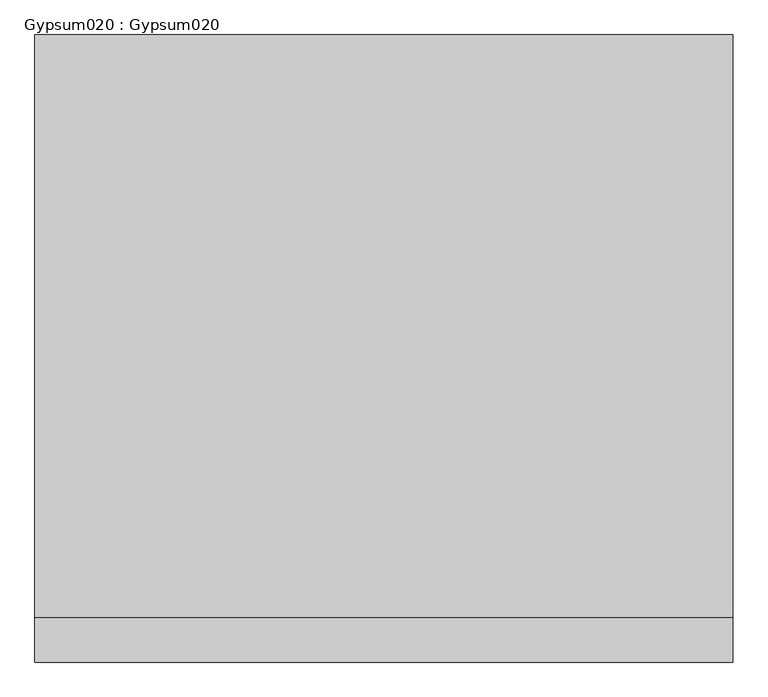
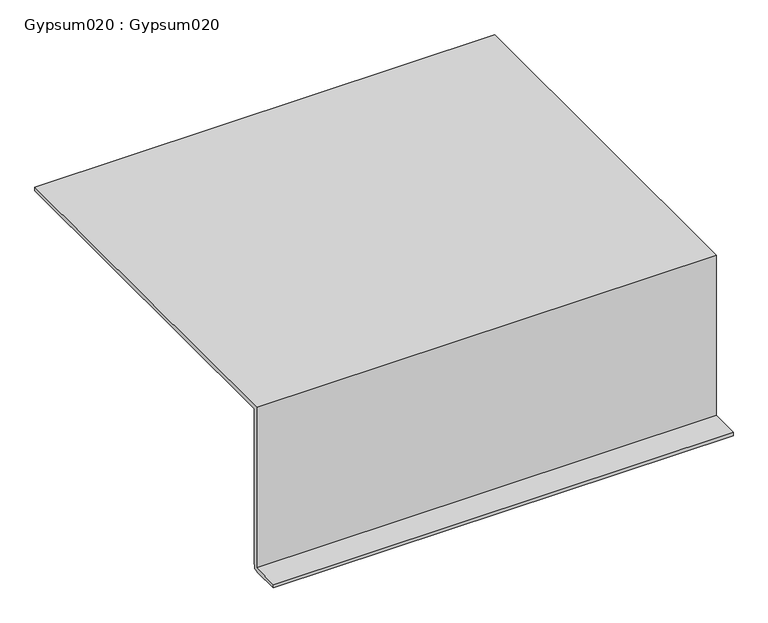
"""IFC4 building model written with IfcOpenShell, lengths in millimetres: proxy geometry, Gypsum020 : Gypsum020."""

from ifc_helpers import new_model, si_unit, frame, origin, place, context, project, spatial, polyline, outline, extrude, source, transform, mapped, element, save


def gypsum020_gypsum020_7a812923(model_context):
    return source(origin(), model_context, "Body", "SweptSolid", [
        extrude(outline(polyline([(-4625.5194659, 39003.2209974), (-4625.5194659, 39019.0959974), (-4497.8425368, 39019.0959974), (-4497.8425368, 39757.096), (-2827.7925368, 39757.096), (-2827.7925368, 39741.221), (-4481.9675368, 39741.221), (-4481.9675368, 39025.6541813), (-4483.2475368, 39025.6541813), (-4483.2475368, 39004.5009974), (-4504.4007207, 39004.5009974), (-4504.4007207, 39003.2209974), (-4625.5194659, 39003.2209974)])), frame((12382.7678845, 0.0, 0.0), z_axis=(1.0, 0.0, 0.0), x_axis=(0.0, 1.0, 0.0)), (0.0, 0.0, 1.0), 2000.0),
    ])


if __name__ == "__main__":
    model = new_model("IFC4")
    model_context = context("Model", 3, world=origin())
    ifc_project = project(units=[si_unit("LENGTHUNIT", "METRE", prefix="MILLI")], contexts=[model_context])
    site = spatial("IfcSite", under=ifc_project)
    building = spatial("IfcBuilding", under=site)
    placement = place(None, origin())
    gypsum020_gypsum020_shape = gypsum020_gypsum020_7a812923(model_context)
    element("IfcBuildingElementProxy", 1, Name="Gypsum020 : Gypsum020", ObjectType="Gypsum020 : Gypsum020", at=placement, inside=building, context=model_context, shape_type="MappedRepresentation", body=[
        mapped(gypsum020_gypsum020_shape, transform((0.0, 0.0, 0.0), x_axis=(1.0, 0.0, 0.0), y_axis=(0.0, 1.0, 0.0), z_axis=(0.0, 0.0, 1.0))),
    ])
    save(model, "model.ifc")

# Revit data of these elements
# Type "Gypsum020 : Gypsum020"
#   NameOverride = "Gypsum020"
# Element 1 (IfcBuildingElementProxy, "Gypsum020 : Gypsum020")
#   Materials on its faces: "5/8\"  GYPSUM BOARD"
# Materials
#   "5/8\"  GYPSUM BOARD": class "Unassigned", colour RGB 255 255 255, transparency 0, Cost = 0
